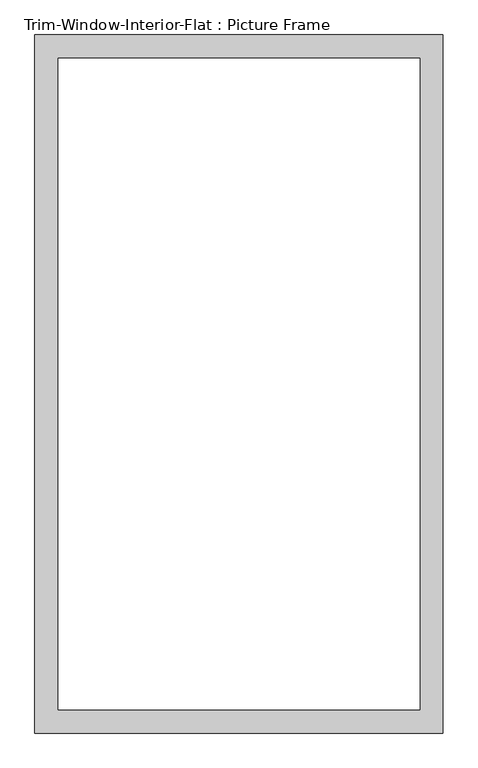
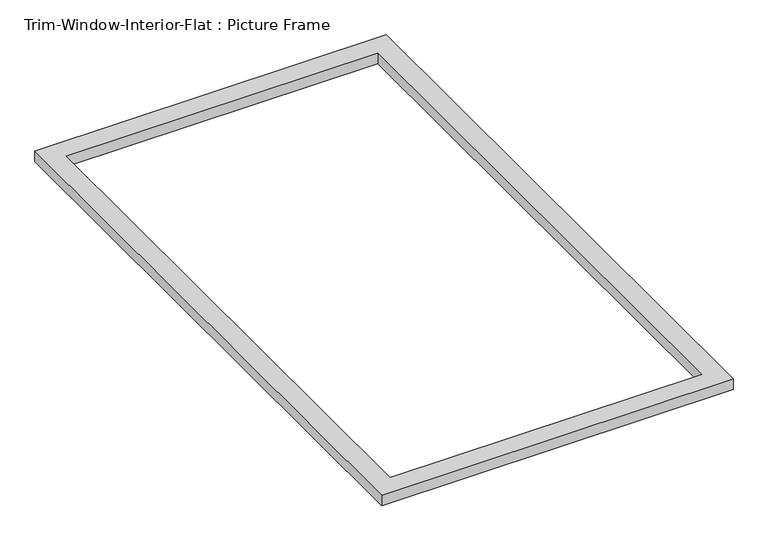
"""IFC4 building model written with IfcOpenShell, lengths in millimetres: proxy geometry, Trim-Window-Interior-Flat : Picture Frame."""

from ifc_helpers import new_model, si_unit, origin, origin_with_axes, place, context, project, spatial, polyline, outline, extrude, source, transform, mapped, element, save


def trim_window_interior_flat_picture_frame_9b9b1be9(model_context):
    return source(origin(), model_context, "Body", "SweptSolid", [
        extrude(outline(polyline([(501.65, 44.45), (501.65, -1670.05), (-501.65, -1670.05), (-501.65, 44.45), (501.65, 44.45)]), holes=[polyline([(444.5, -12.7), (-444.5, -12.7), (-444.5, -1612.9), (444.5, -1612.9), (444.5, -12.7)])]), origin_with_axes(), (0.0, 0.0, 1.0), 31.75),
    ])


if __name__ == "__main__":
    model = new_model("IFC4")
    model_context = context("Model", 3, world=origin())
    ifc_project = project(units=[si_unit("LENGTHUNIT", "METRE", prefix="MILLI")], contexts=[model_context])
    site = spatial("IfcSite", under=ifc_project)
    building = spatial("IfcBuilding", under=site)
    placement = place(None, origin())
    trim_window_interior_flat_picture_frame_shape = trim_window_interior_flat_picture_frame_9b9b1be9(model_context)
    element("IfcBuildingElementProxy", 1, Name="Trim-Window-Interior-Flat : Picture Frame", ObjectType="Trim-Window-Interior-Flat : Picture Frame", at=placement, inside=building, context=model_context, shape_type="MappedRepresentation", body=[
        mapped(trim_window_interior_flat_picture_frame_shape, transform((0.0, 0.0, 0.0), x_axis=(1.0, 0.0, 0.0), y_axis=(0.0, 1.0, 0.0), z_axis=(0.0, 0.0, 1.0))),
    ])
    save(model, "model.ifc")

# Revit data of these elements
# Type "Trim-Window-Interior-Flat : Picture Frame"
#   Trim Thickness_Picture Frame = 0' - 1 1/4"
#   Trim Width = 0' - 2 1/4"
#   Trim Thickness_with Sill = 0' - 0 3/4"
#   Sill Thickness = 0' - 1 1/4"
#   Opening Width [instance default] = 2' - 0"
#   Opening Height [instance default] = 3' - 0"
#   Default Elevation = 4' - 0"
#   Sill = no
#   Picture Frame = yes
#   Trim Material [instance default] = none
# Element 1 (IfcBuildingElementProxy, "Trim-Window-Interior-Flat : Picture Frame")
#   Opening Width = 3' - 0"
#   Opening Height = 5' - 4"
#   Trim Material = Wood - Stained
#   Materials on its faces: "Wood - Stained"
# Materials
#   "Wood - Stained": class "Wood", colour RGB 224 178 126, transparency 0, Cost = 0
